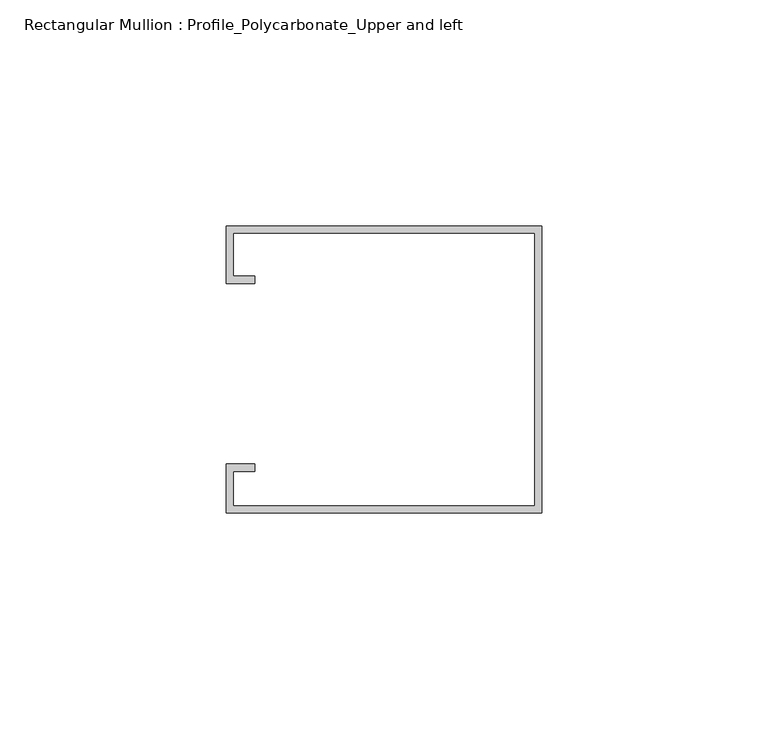
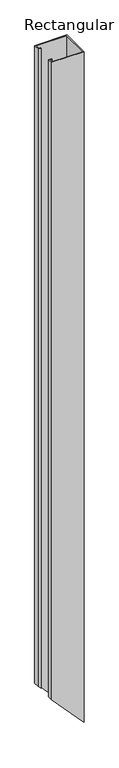
"""IFC4 building model written with IfcOpenShell, lengths in millimetres: member geometry, Rectangular Mullion : Profile_Polycarbonate_Upper and left."""

from ifc_helpers import new_model, si_unit, origin, place, context, project, spatial, faceted_brep, source, transform, mapped, element, save


def rectangular_mullion_profile_polycarbonate_upper_and_left_b0e57842(model_context):
    return source(origin(), model_context, "Body", "Brep", [
        faceted_brep([(0.0, 32.7, 0.0), (-69.85, 32.7, 0.0), (-69.85, 20.0, 0.0), (-63.5, 20.0, 0.0), (-63.5, 21.5875, 0.0), (-68.2625, 21.5875, 0.0), (-68.2625, 31.1125, 0.0), (-1.5875, 31.1125, 0.0), (-1.5875, -29.2125, 0.0), (-68.2625, -29.2125, 0.0), (-68.2625, -21.5875, 0.0), (-63.5, -21.5875, 0.0), (-63.5, -20.0, 0.0), (-69.85, -20.0, 0.0), (-69.85, -30.8, 0.0), (0.0, -30.8, 0.0), (0.0, 32.7, -1532.0697917), (-69.85, 32.7, -1456.1568432), (-69.85, 20.0, -1456.1568432), (-63.5, 20.0, -1463.0580204), (-63.5, 21.5875, -1463.0580204), (-68.2625, 21.5875, -1457.8821375), (-68.2625, 31.1125, -1457.8821375), (-1.5875, 31.1125, -1530.3444974), (-1.5875, -29.2125, -1530.3444974), (-68.2625, -29.2125, -1457.8821375), (-68.2625, -21.5875, -1457.8821375), (-63.5, -21.5875, -1463.0580204), (-63.5, -20.0, -1463.0580204), (-69.85, -20.0, -1456.1568432), (-69.85, -30.8, -1456.1568432), (0.0, -30.8, -1532.0697917)], [[[0, 1, 2, 3, 4, 5, 6, 7, 8, 9, 10, 11, 12, 13, 14, 15]], [[1, 0, 16, 17]], [[2, 1, 17, 18]], [[3, 2, 18, 19]], [[4, 3, 19, 20]], [[5, 4, 20, 21]], [[6, 5, 21, 22]], [[7, 6, 22, 23]], [[8, 7, 23, 24]], [[9, 8, 24, 25]], [[10, 9, 25, 26]], [[11, 10, 26, 27]], [[12, 11, 27, 28]], [[13, 12, 28, 29]], [[14, 13, 29, 30]], [[15, 14, 30, 31]], [[0, 15, 31, 16]], [[16, 31, 30, 29, 28, 27, 26, 25, 24, 23, 22, 21, 20, 19, 18, 17]]]),
    ])


if __name__ == "__main__":
    model = new_model("IFC4")
    model_context = context("Model", 3, world=origin())
    ifc_project = project(units=[si_unit("LENGTHUNIT", "METRE", prefix="MILLI")], contexts=[model_context])
    site = spatial("IfcSite", under=ifc_project)
    building = spatial("IfcBuilding", under=site)
    placement = place(None, origin())
    rectangular_mullion_profile_polycarbonate_upper_and_left_shape = rectangular_mullion_profile_polycarbonate_upper_and_left_b0e57842(model_context)
    element("IfcMember", 1, ObjectType="Rectangular Mullion : Profile_Polycarbonate_Upper and left", at=placement, inside=building, context=model_context, shape_type="MappedRepresentation", body=[
        mapped(rectangular_mullion_profile_polycarbonate_upper_and_left_shape, transform((0.0, 0.0, 0.0), x_axis=(1.0, 0.0, 0.0), y_axis=(0.0, 1.0, 0.0), z_axis=(0.0, 0.0, 1.0))),
    ])
    save(model, "model.ifc")

# Revit data of these elements
# Type "Rectangular Mullion : Profile_Polycarbonate_Upper and left"
#   built-in parameter 1007322 = 0.208333 (stored number, unit not read)
#   built-in parameter 1007321 = 0.00520833 (stored number, unit not read)
#   built-in parameter 1007320 = 0 (stored number, unit not read)
# Element 1 (IfcMember, "Rectangular Mullion : Profile_Polycarbonate_Upper and left")
#   Materials on its faces: "ALUMINUM PROFILE AT POLYCARBONATE PANEL"
# Materials
#   "ALUMINUM PROFILE AT POLYCARBONATE PANEL": class "Metal", colour RGB 244 244 244, transparency 0, Description = "Aluminum 6061", Cost = 0
